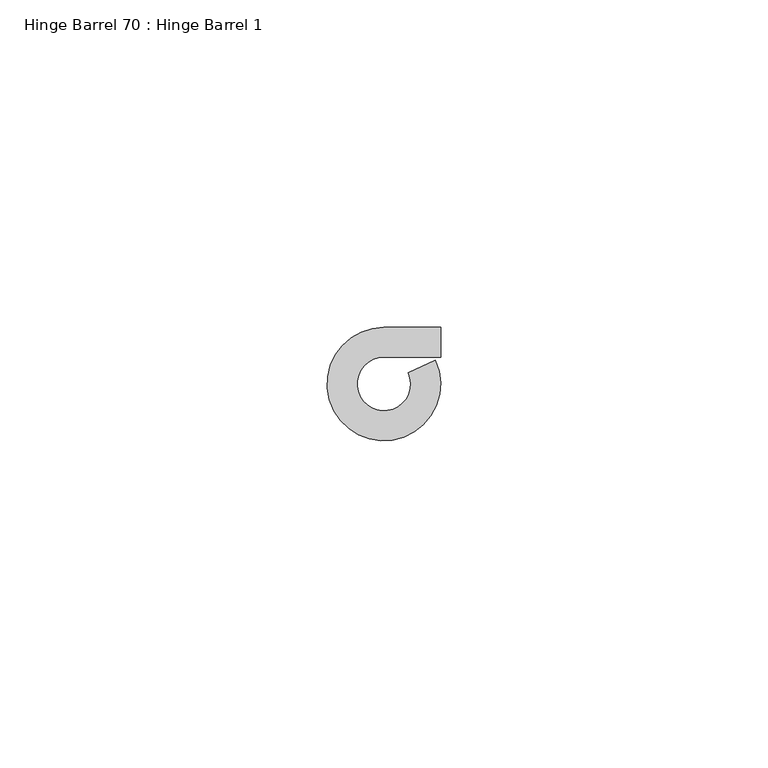
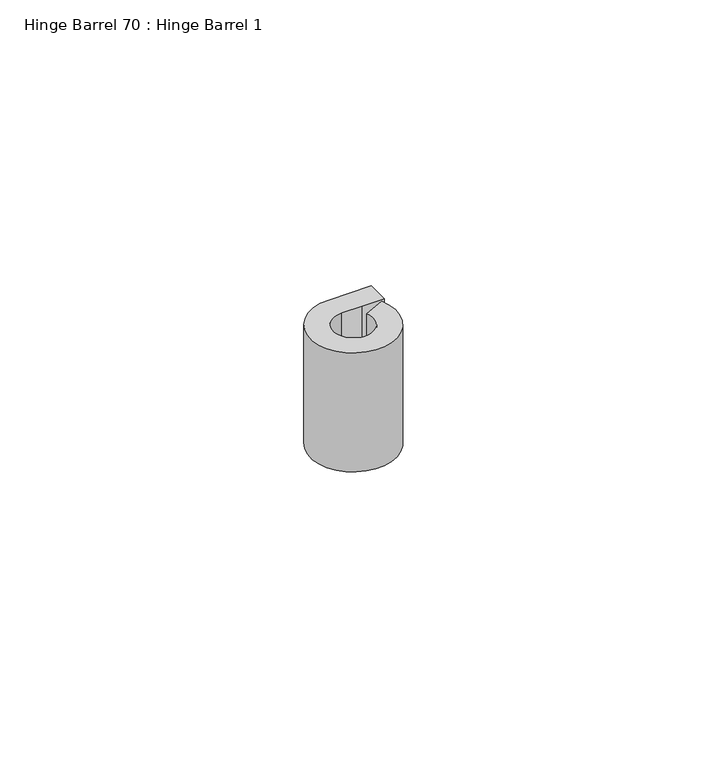
"""IFC4 building model written with IfcOpenShell, lengths in millimetres: proxy geometry, Hinge Barrel 70 : Hinge Barrel 1."""

from ifc_helpers import new_model, si_unit, point, frame, frame_2d, origin, place, context, project, spatial, polyline, circle_curve, trimmed, segment, composite_curve, outline, extrude, source, transform, mapped, element, save


def hinge_barrel_70_hinge_barrel_1_c7bfcbc0(model_context):
    return source(origin(), model_context, "Body", "SweptSolid", [
        extrude(outline(composite_curve([segment(polyline([(587323.2214739, -536306.2758841), (587319.1320739, -536306.2758841)]), True, "CONTINUOUS"), segment(trimmed(circle_curve(frame_2d((587319.1320739, -536310.3652841)), 4.0894), [point((587319.1320739, -536306.2758841))], [point((587322.8436736, -536308.6485371))], True, "CARTESIAN"), True, "CONTINUOUS"), segment(polyline([(587322.8436736, -536308.6485371), (587326.986084, -536306.7325249)]), True, "CONTINUOUS"), segment(trimmed(circle_curve(frame_2d((587319.1320739, -536310.3652841)), 8.6534625), [point((587326.986084, -536306.7325249))], [point((587319.1320739, -536301.7118216))], False, "CARTESIAN"), True, "CONTINUOUS"), segment(polyline([(587319.1320739, -536301.7118216), (587327.7934739, -536301.7118216), (587327.7934739, -536306.2758841), (587323.2214739, -536306.2758841)]), True, "CONTINUOUS")], self_intersect=False)), frame((0.0, 0.0, 1225.55), z_axis=(0.0, 0.0, 1.0), x_axis=(1.0, 0.0, 0.0)), (0.0, 0.0, 1.0), 25.4),
    ])


if __name__ == "__main__":
    model = new_model("IFC4")
    model_context = context("Model", 3, world=origin())
    ifc_project = project(units=[si_unit("LENGTHUNIT", "METRE", prefix="MILLI")], contexts=[model_context])
    site = spatial("IfcSite", under=ifc_project)
    building = spatial("IfcBuilding", under=site)
    placement = place(None, origin())
    hinge_barrel_70_hinge_barrel_1_shape = hinge_barrel_70_hinge_barrel_1_c7bfcbc0(model_context)
    element("IfcBuildingElementProxy", 1, Name="Hinge Barrel 70 : Hinge Barrel 1", ObjectType="Hinge Barrel 70 : Hinge Barrel 1", at=placement, inside=building, context=model_context, shape_type="MappedRepresentation", body=[
        mapped(hinge_barrel_70_hinge_barrel_1_shape, transform((0.0, 0.0, 0.0), x_axis=(1.0, 0.0, 0.0), y_axis=(0.0, 1.0, 0.0), z_axis=(0.0, 0.0, 1.0))),
    ])
    save(model, "model.ifc")

# Revit data of these elements
# Element 1 (IfcBuildingElementProxy, "Hinge Barrel 70 : Hinge Barrel 1")
#   Materials on its faces: "6\"X6\" WELD-ON STL BUTT HINGE"
# Materials
#   "6\"X6\" WELD-ON STL BUTT HINGE": class "Metal", colour RGB 189 187 185, transparency 0, Description = "Carbon steel", Cost = 0
